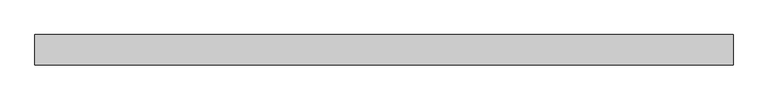
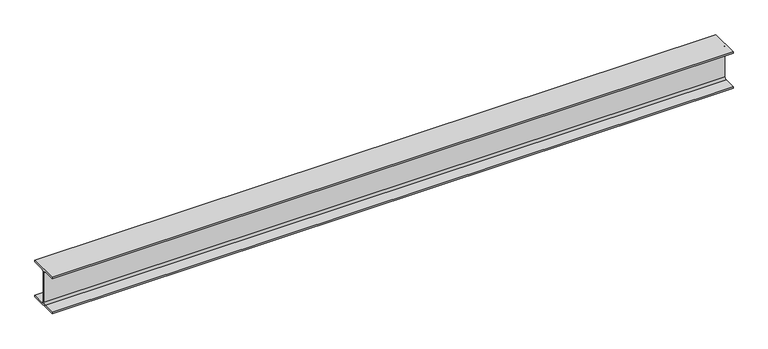
"""IFC4 building model written with IfcOpenShell, lengths in millimetres: beam geometry, 0912_Steel Framing_H-KSD3502 : H_SB_ASB_H-390x300x10x16."""

from ifc_helpers import new_model, si_unit, point, frame, frame_2d, origin, place, context, project, spatial, polyline, circle_curve, trimmed, segment, composite_curve, outline, extrude, source, transform, mapped, element, save


def beam_4e65f60f(model_context):
    return source(origin(), model_context, "Body", "SweptSolid", [
        extrude(outline(composite_curve([segment(polyline([(150.0, -179.0), (150.0, -195.0), (-150.0, -195.0), (-150.0, -179.0), (-27.0, -179.0)]), True, "CONTINUOUS"), segment(trimmed(circle_curve(frame_2d((-27.0, -157.0)), 22.0), [point((-27.0, -179.0))], [point((-5.0, -157.0))], True, "CARTESIAN"), True, "CONTINUOUS"), segment(polyline([(-5.0, -157.0), (-5.0, 157.0)]), True, "CONTINUOUS"), segment(trimmed(circle_curve(frame_2d((-27.0, 157.0)), 22.0), [point((-5.0, 157.0))], [point((-27.0, 179.0))], True, "CARTESIAN"), True, "CONTINUOUS"), segment(polyline([(-27.0, 179.0), (-150.0, 179.0), (-150.0, 195.0), (150.0, 195.0), (150.0, 179.0), (27.0, 179.0)]), True, "CONTINUOUS"), segment(trimmed(circle_curve(frame_2d((27.0, 157.0)), 22.0), [point((27.0, 179.0))], [point((5.0, 157.0))], True, "CARTESIAN"), True, "CONTINUOUS"), segment(polyline([(5.0, 157.0), (5.0, -157.0)]), True, "CONTINUOUS"), segment(trimmed(circle_curve(frame_2d((27.0, -157.0)), 22.0), [point((5.0, -157.0))], [point((27.0, -179.0))], True, "CARTESIAN"), True, "CONTINUOUS"), segment(polyline([(27.0, -179.0), (150.0, -179.0)]), True, "CONTINUOUS")], self_intersect=False)), frame((-3404.8, 0.0, 0.0), z_axis=(1.0, 0.0, 0.0), x_axis=(0.0, 1.0, 0.0)), (0.0, 0.0, 1.0), 6892.0999994),
    ])


if __name__ == "__main__":
    model = new_model("IFC4")
    model_context = context("Model", 3, world=origin())
    ifc_project = project(units=[si_unit("LENGTHUNIT", "METRE", prefix="MILLI")], contexts=[model_context])
    site = spatial("IfcSite", under=ifc_project)
    building = spatial("IfcBuilding", under=site)
    placement = place(None, origin())
    beam_shape = beam_4e65f60f(model_context)
    element("IfcBeam", 1, ObjectType="0912_Steel Framing_H-KSD3502 : H_SB_ASB_H-390x300x10x16", at=placement, inside=building, context=model_context, shape_type="MappedRepresentation", body=[
        mapped(beam_shape, transform((0.0, 0.0, 0.0), x_axis=(1.0, 0.0, 0.0), y_axis=(0.0, 1.0, 0.0), z_axis=(0.0, 0.0, 1.0))),
    ])
    save(model, "model.ifc")

# Revit data of these elements
# Type "0912_Steel Framing_H-KSD3502 : H_SB_ASB_H-390x300x10x16"
#   H_WM Code_1 = "S01AA001-00001 | Main Steel Structure Fabrication Work | Shelter/Building | Heavy Steel - Standard (Weight≥90KG/M) | Material: (   )"
#   H_WM Code_2 = "S03AA027-00001 | Main Steel Structure Erection Work | Shelter/Building | Heavy Steel (Weight≥90KG/M) | Material: (   )"
#   H_WM Code_3 = "S01AA010-00001 | Main Steel Structure Fabrication Work | Shelter/Building | Steel Painting/Coating | for Non-Fireproofed Steel Surface, Surface Preparation, Primer, Second & Final Coat | Material: (   )"
#   H_Q'ty Cal Type Tag = "SB-Q2"
#   Width = 30.0 cm
#   Web Thickness = 1.0 cm
#   Web Fillet = 2.2 cm
#   Warping Constant = 2520000.0 cm⁶
#   W = 0
#   Torsional Moment of Inertia = 94.3867 cm⁴
#   Section Area = 136.0 cm²
#   Plastic Modulus weak axis = 733.0 cm³
#   Plastic Modulus strong axis = 2190.0 cm³
#   Perimeter = 1.92 m²/m
#   Nominal Weight = 107.00 kgf/m
#   Moment of Inertia weak axis = 7210.00 cm⁴
#   Moment of Inertia strong axis = 38700.00 cm⁴
#   Height = 39.0 cm
#   Flange Thickness = 1.6 cm
#   Elastic Modulus weak axis = 481.0 cm³
#   Elastic Modulus strong axis = 1980.0 cm³
#   Centroid Vertical = 19.5 cm
#   Centroid Horizontal = 15.0 cm
#   Ix = 387000000
#   Length [instance default] = 1.5240 m
#   Zx = 2190000
#   b = 0.3000 m
#   h = 0.3900 m
#   r = 0.0220 m
#   s = 0.0100 m
#   t = 0.0160 m
#   A = 0.0136 m²
#   Structural Material [instance default] = Steel, 45-345
#   Assembly Code = ""
# Element 1 (IfcBeam, "0912_Steel Framing_H-KSD3502 : H_SB_ASB_H-390x300x10x16")
#   Structural Material = none
# Materials
#   "Steel, 45-345": class "Metal", colour RGB 189 187 185, transparency 0, Description = "Steel 345 MPa", Cost = 0
